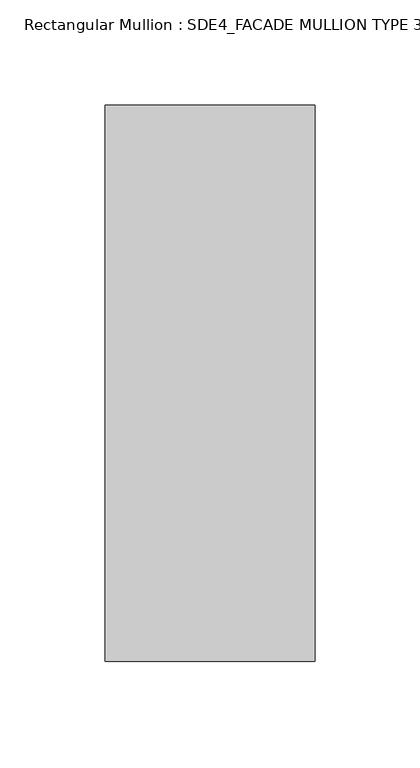
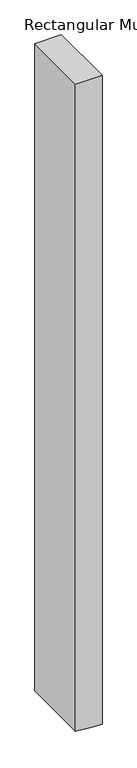
"""IFC4 building model written with IfcOpenShell, lengths in millimetres: member geometry, Rectangular Mullion : SDE4_FACADE MULLION TYPE 3."""

from ifc_helpers import new_model, si_unit, frame, origin, place, context, project, spatial, polyline, outline, extrude, source, transform, mapped, element, save


def rectangular_mullion_sde4_facade_mullion_type_3_b86b561e(model_context):
    return source(origin(), model_context, "Body", "SweptSolid", [
        extrude(outline(polyline([(0.0, 50.0), (0.0, -50.0), (-2579.3401079, -50.0), (-2583.406187, 3.056508), (-2587.0037843, 50.0), (0.0, 50.0)])), frame((0.0, -132.5, 0.0), z_axis=(0.0, 1.0, 0.0), x_axis=(0.0, 0.0, 1.0)), (0.0, 0.0, 1.0), 265.0),
    ])


if __name__ == "__main__":
    model = new_model("IFC4")
    model_context = context("Model", 3, world=origin())
    ifc_project = project(units=[si_unit("LENGTHUNIT", "METRE", prefix="MILLI")], contexts=[model_context])
    site = spatial("IfcSite", under=ifc_project)
    building = spatial("IfcBuilding", under=site)
    placement = place(None, origin())
    rectangular_mullion_sde4_facade_mullion_type_3_shape = rectangular_mullion_sde4_facade_mullion_type_3_b86b561e(model_context)
    element("IfcMember", 1, ObjectType="Rectangular Mullion : SDE4_FACADE MULLION TYPE 3", at=placement, inside=building, context=model_context, shape_type="MappedRepresentation", body=[
        mapped(rectangular_mullion_sde4_facade_mullion_type_3_shape, transform((0.0, 0.0, 0.0), x_axis=(1.0, 0.0, 0.0), y_axis=(0.0, 1.0, 0.0), z_axis=(0.0, 0.0, 1.0))),
    ])
    save(model, "model.ifc")

# Revit data of these elements
# Type "Rectangular Mullion : SDE4_FACADE MULLION TYPE 3"
#   built-in parameter 1007322 = 0.869423 (stored number, unit not read)
#   built-in parameter 1007321 = 0.164042 (stored number, unit not read)
#   built-in parameter 1007320 = 0.164042 (stored number, unit not read)
